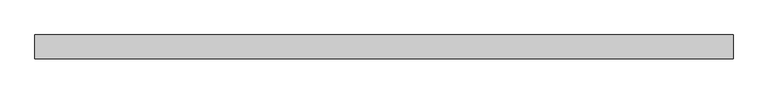
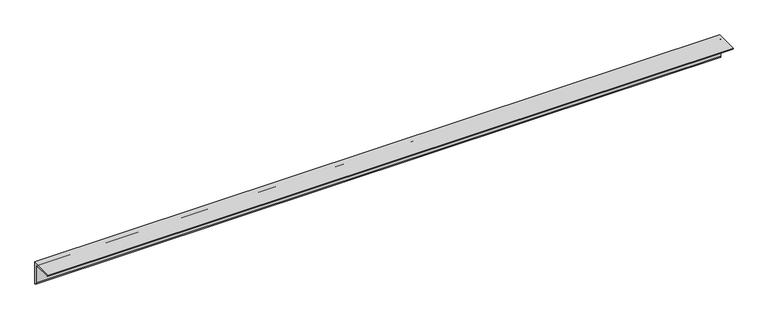
"""IFC4 building model written with IfcOpenShell, lengths in millimetres: member geometry, 0912_Steel Framing_L-KSD3502 : H_SB_AR_S03_L-130x130x12_HBR3."""

from ifc_helpers import new_model, si_unit, point, frame, frame_2d, origin, place, context, project, spatial, polyline, circle_curve, trimmed, segment, composite_curve, outline, extrude, source, transform, mapped, element, save


def member_00a8a024(model_context):
    return source(origin(), model_context, "Body", "SweptSolid", [
        extrude(outline(composite_curve([segment(polyline([(36.4, 36.4), (36.4, -93.6)]), True, "CONTINUOUS"), segment(trimmed(circle_curve(frame_2d((36.4, -81.6)), 12.0), [point((36.4, -93.6))], [point((24.4, -81.6))], False, "CARTESIAN"), True, "CONTINUOUS"), segment(polyline([(24.4, -81.6), (24.4, 12.4)]), True, "CONTINUOUS"), segment(trimmed(circle_curve(frame_2d((12.4, 12.4)), 12.0), [point((24.4, 12.4))], [point((12.4, 24.4))], True, "CARTESIAN"), True, "CONTINUOUS"), segment(polyline([(12.4, 24.4), (-81.6, 24.4)]), True, "CONTINUOUS"), segment(trimmed(circle_curve(frame_2d((-81.6, 36.4)), 12.0), [point((-81.6, 24.4))], [point((-93.6, 36.4))], False, "CARTESIAN"), True, "CONTINUOUS"), segment(polyline([(-93.6, 36.4), (36.4, 36.4)]), True, "CONTINUOUS")], self_intersect=False)), frame((-1902.3310425, 0.0, 0.0), z_axis=(1.0, 0.0, 0.0), x_axis=(0.0, 1.0, 0.0)), (0.0, 0.0, 1.0), 3825.3920289),
    ])


if __name__ == "__main__":
    model = new_model("IFC4")
    model_context = context("Model", 3, world=origin())
    ifc_project = project(units=[si_unit("LENGTHUNIT", "METRE", prefix="MILLI")], contexts=[model_context])
    site = spatial("IfcSite", under=ifc_project)
    building = spatial("IfcBuilding", under=site)
    placement = place(None, origin())
    member_shape = member_00a8a024(model_context)
    element("IfcMember", 1, ObjectType="0912_Steel Framing_L-KSD3502 : H_SB_AR_S03_L-130x130x12_HBR3", at=placement, inside=building, context=model_context, shape_type="MappedRepresentation", body=[
        mapped(member_shape, transform((0.0, 0.0, 0.0), x_axis=(1.0, 0.0, 0.0), y_axis=(0.0, 1.0, 0.0), z_axis=(0.0, 0.0, 1.0))),
    ])
    save(model, "model.ifc")

# Revit data of these elements
# Type "0912_Steel Framing_L-KSD3502 : H_SB_AR_S03_L-130x130x12_HBR3"
#   k = 25 mm
#   Perimeter = 0.52 m²/m
#   Nominal Weight = 23.40 kgf/m
#   Length [instance default] = 1000 mm
#   b = 130 mm
#   d = 130 mm
#   t = 12 mm
#   x = 36.4 mm
#   y = 36.4 mm
#   A = 2976.00 m²
#   Structural Material [instance default] = Steel, 45-345
# Element 1 (IfcMember, "0912_Steel Framing_L-KSD3502 : H_SB_AR_S03_L-130x130x12_HBR3")
#   Structural Material = Steel ASTM A36
#   Materials on its faces: "Steel ASTM A36"
# Materials
#   "Steel, 45-345": class "Metal", colour RGB 189 187 185, transparency 0, Description = "Steel 345 MPa", Cost = 0
#   "Steel ASTM A36": class "Metal", colour RGB 199 199 199, transparency 0, Description = "Structural steel, ASTM A36 Grade B, mill finish", Cost = 0
